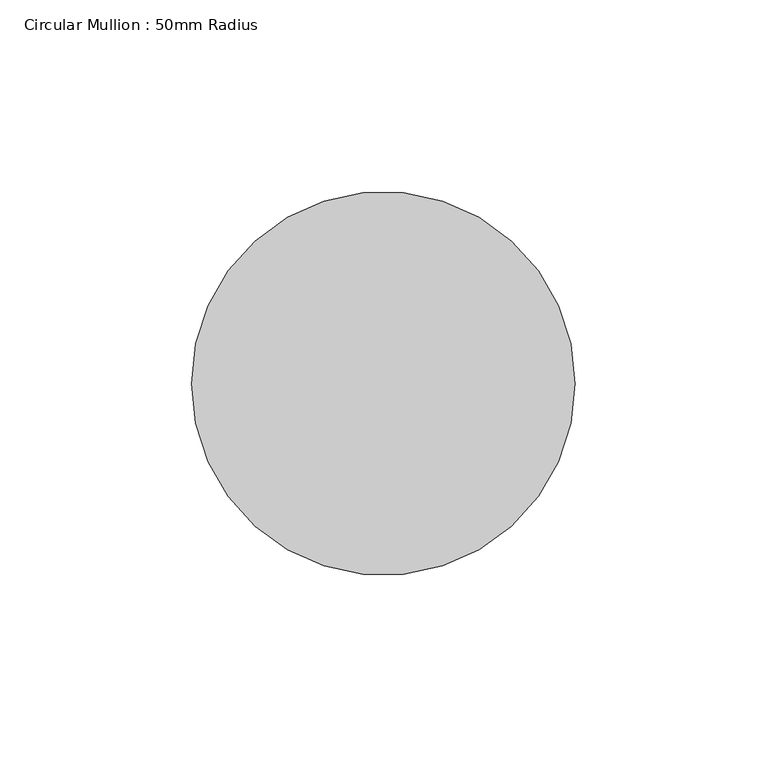
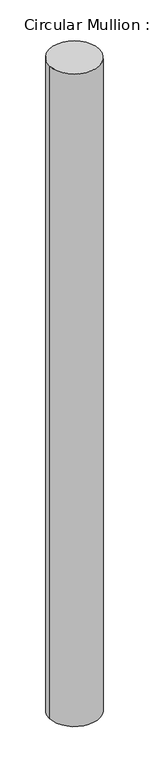
"""IFC4 building model written with IfcOpenShell, lengths in millimetres: member geometry, Circular Mullion : 50mm Radius."""

import ifcopenshell
import ifcopenshell.guid

model = None  # the IFC model being written
_history = None  # IfcOwnerHistory: only IFC2X3 demands one
_inside = {}  # id of a spatial element -> (the spatial element, [elements in it])
_under = {}  # id of a project, library or spatial element -> (it, [spatial elements below it])
_declared = {}  # id of a project -> (the project, [libraries it declares])
_typed = {}  # id of a type object -> (the type object, [elements of that type])
_made_of = {}  # id of a material, layer set ... -> (it, [elements and type objects made of it])


def new_model(schema):
    """Start an empty IFC model of exactly this schema.

    Asked for "IFC4X3", IfcOpenShell would pick the latest addendum, in which some entities
    have other attributes; the version numbers below select the first issue.
    IFC2X3 requires an IfcOwnerHistory on every rooted entity: one is made here for all.
    """
    global model, _history
    if schema == "IFC4X3":
        model = ifcopenshell.file(schema_version=(4, 3, 0, 0))
    else:
        model = ifcopenshell.file(schema=schema)
    _inside.clear()
    _under.clear()
    _declared.clear()
    _typed.clear()
    _made_of.clear()
    _history = None
    if model.schema == "IFC2X3":
        org = make("IfcOrganization", Name="unknown")
        user = make(
            "IfcPersonAndOrganization",
            ThePerson=make("IfcPerson", FamilyName="unknown"),
            TheOrganization=org,
        )
        app = make(
            "IfcApplication",
            ApplicationDeveloper=org,
            Version="unknown",
            ApplicationFullName="unknown",
            ApplicationIdentifier="unknown",
        )
        _history = make(
            "IfcOwnerHistory",
            OwningUser=user,
            OwningApplication=app,
            ChangeAction="ADDED",
            CreationDate=0,
        )
    return model


def make(cls, **values):
    """One entity of the class cls with the attributes given. An attribute that is None is left unset."""
    return model.create_entity(
        cls, **{name: value for name, value in values.items() if value is not None}
    )


def rooted(cls, **values):
    """An entity with a GlobalId (a new one), such as an element, a storey or a relation."""
    return make(cls, GlobalId=ifcopenshell.guid.new(), OwnerHistory=_history, **values)


def si_unit(unit_type, name, prefix=None):
    """IfcSIUnit, for example si_unit("LENGTHUNIT", "METRE", prefix="MILLI")."""
    return make("IfcSIUnit", UnitType=unit_type, Prefix=prefix, Name=name)


def assignment(units):
    """IfcUnitAssignment: the units of a project."""
    return None if units is None else make("IfcUnitAssignment", Units=units)


def point(xyz):
    """IfcCartesianPoint."""
    return None if xyz is None else make("IfcCartesianPoint", Coordinates=xyz)


def direction(xyz):
    """IfcDirection."""
    return None if xyz is None else make("IfcDirection", DirectionRatios=xyz)


def frame(location, z_axis=None, x_axis=None):
    """IfcAxis2Placement3D, a coordinate frame: its origin and axes. An axis left out is left unset."""
    return make(
        "IfcAxis2Placement3D",
        Location=point(location),
        Axis=direction(z_axis),
        RefDirection=direction(x_axis),
    )


def frame_2d(location, x_axis=None):
    """IfcAxis2Placement2D, a coordinate frame in the plane: its origin and x axis."""
    return make(
        "IfcAxis2Placement2D", Location=point(location), RefDirection=direction(x_axis)
    )


def origin():
    """The frame at (0, 0, 0) with its axes left unset."""
    return frame((0.0, 0.0, 0.0))


def origin_2d():
    """The frame at (0, 0) in the plane with its x axis left unset."""
    return frame_2d((0.0, 0.0))


def place(relative_to, where):
    """IfcLocalPlacement: puts the frame where relative to a parent placement (None: the world)."""
    return make(
        "IfcLocalPlacement", PlacementRelTo=relative_to, RelativePlacement=where
    )


def context(
    kind, dimensions, precision=None, world=None, true_north=None, identifier=None
):
    """IfcGeometricRepresentationContext, for example the 3D "Model" context."""
    return make(
        "IfcGeometricRepresentationContext",
        ContextIdentifier=identifier,
        ContextType=kind,
        CoordinateSpaceDimension=dimensions,
        Precision=precision,
        WorldCoordinateSystem=world,
        TrueNorth=true_north,
    )


def project(units=None, contexts=None):
    """IfcProject with its units and contexts."""
    return rooted(
        "IfcProject",
        Name="project",
        RepresentationContexts=contexts,
        UnitsInContext=assignment(units),
    )


def spatial(cls, under=None, at=None, **own):
    """A site, building, storey or space (cls), placed at a placement, below another one or the project."""
    s = rooted(cls, ObjectPlacement=at, **own)
    if under is not None:
        _under.setdefault(under.id(), (under, []))[1].append(s)
    return s


def circle_curve(where, radius):
    """IfcCircle in the frame where."""
    return make("IfcCircle", Position=where, Radius=radius)


def trimmed(basis, trim1, trim2, sense, master):
    """IfcTrimmedCurve: the piece of a basis curve between two trims."""
    return make(
        "IfcTrimmedCurve",
        BasisCurve=basis,
        Trim1=trim1,
        Trim2=trim2,
        SenseAgreement=sense,
        MasterRepresentation=master,
    )


def segment(curve, same_sense, transition):
    """IfcCompositeCurveSegment."""
    return make(
        "IfcCompositeCurveSegment",
        Transition=transition,
        SameSense=same_sense,
        ParentCurve=curve,
    )


def composite_curve(segments, self_intersect=None):
    """IfcCompositeCurve: segments joined end to end."""
    return make("IfcCompositeCurve", Segments=segments, SelfIntersect=self_intersect)


def outline(outer, holes=None, kind="AREA"):
    """IfcArbitraryClosedProfileDef: a profile drawn as a closed curve; with holes, ...WithVoids."""
    if holes is None:
        return make("IfcArbitraryClosedProfileDef", ProfileType=kind, OuterCurve=outer)
    return make(
        "IfcArbitraryProfileDefWithVoids",
        ProfileType=kind,
        OuterCurve=outer,
        InnerCurves=holes,
    )


def extrude(swept, where, along, depth):
    """IfcExtrudedAreaSolid: the profile swept, set in the frame where, extruded along a direction by depth."""
    return make(
        "IfcExtrudedAreaSolid",
        SweptArea=swept,
        Position=where,
        ExtrudedDirection=direction(along),
        Depth=depth,
    )


def shape(context_of_items, identifier, shape_type, items):
    """IfcShapeRepresentation: the items that make up one representation, for example the "Body"."""
    return make(
        "IfcShapeRepresentation",
        ContextOfItems=context_of_items,
        RepresentationIdentifier=identifier,
        RepresentationType=shape_type,
        Items=items,
    )


def source(mapping_origin, context_of_items, identifier, shape_type, items):
    """IfcRepresentationMap: a shape defined once, which mapped items show again and again."""
    return make(
        "IfcRepresentationMap",
        MappingOrigin=mapping_origin,
        MappedRepresentation=shape(context_of_items, identifier, shape_type, items),
    )


def transform(
    local_origin,
    x_axis=None,
    y_axis=None,
    z_axis=None,
    scale=None,
    scale2=None,
    scale3=None,
    uniform=True,
):
    """IfcCartesianTransformationOperator3D, or its non-uniform kind. x_axis, y_axis, z_axis: its Axis1, 2, 3."""
    if uniform:
        return make(
            "IfcCartesianTransformationOperator3D",
            Axis1=direction(x_axis),
            Axis2=direction(y_axis),
            LocalOrigin=point(local_origin),
            Scale=scale,
            Axis3=direction(z_axis),
        )
    return make(
        "IfcCartesianTransformationOperator3DnonUniform",
        Axis1=direction(x_axis),
        Axis2=direction(y_axis),
        LocalOrigin=point(local_origin),
        Scale=scale,
        Axis3=direction(z_axis),
        Scale2=scale2,
        Scale3=scale3,
    )


def mapped(mapping_source, mapping_target):
    """IfcMappedItem: shows the shape of a source again, moved by a transform."""
    return make(
        "IfcMappedItem", MappingSource=mapping_source, MappingTarget=mapping_target
    )


def made_of(thing, what):
    """Note that an element or type object is made of a material, layer set ...; save() writes the relation."""
    if what is not None:
        _made_of.setdefault(what.id(), (what, []))[1].append(thing)
    return thing


def element(
    cls,
    number,
    at=None,
    inside=None,
    cuts=None,
    type_object=None,
    material=None,
    context=None,
    identifier="Body",
    shape_type=None,
    held_by="IfcProductDefinitionShape",
    body=None,
    shapes=None,
    **own,
):
    """One element of the class cls, such as IfcWall. Its Tag is "e" and its number.

    at: its placement. inside: the storey or other place that contains it. cuts: it is an
    opening in that element (IfcRelVoidsElement). A single representation is given by context,
    identifier, shape_type and body (its items); several are given by shapes. held_by: the class
    of the entity that holds the representations. save() writes the other relations.
    """
    e = rooted(cls, Tag="e%d" % number, ObjectPlacement=at, **own)
    if body is not None:
        shapes = [shape(context, identifier, shape_type, body)]
    if shapes is not None:
        e.Representation = make(held_by, Representations=shapes)
    if inside is not None:
        _inside.setdefault(inside.id(), (inside, []))[1].append(e)
    if cuts is not None:
        rooted(
            "IfcRelVoidsElement", RelatingBuildingElement=cuts, RelatedOpeningElement=e
        )
    if type_object is not None:
        _typed.setdefault(type_object.id(), (type_object, []))[1].append(e)
    return made_of(e, material)


def aggregate(whole, parts):
    """IfcRelAggregates: a whole, such as a stair, and the parts it consists of."""
    return rooted("IfcRelAggregates", RelatingObject=whole, RelatedObjects=parts)


def save(model, path):
    """Write the relations noted so far, then the file.

    IfcRelAggregates (storeys below a building ...), IfcRelContainedInSpatialStructure (elements
    in a storey), IfcRelDefinesByType, IfcRelAssociatesMaterial and IfcRelDeclares: one each for
    every whole, place, type object, material and project.
    """
    for whole, parts in _under.values():
        aggregate(whole, parts)
    for where, things in _inside.values():
        rooted(
            "IfcRelContainedInSpatialStructure",
            RelatedElements=things,
            RelatingStructure=where,
        )
    for kind, things in _typed.values():
        rooted("IfcRelDefinesByType", RelatedObjects=things, RelatingType=kind)
    for what, things in _made_of.values():
        rooted("IfcRelAssociatesMaterial", RelatedObjects=things, RelatingMaterial=what)
    for by, libraries in _declared.values():
        rooted("IfcRelDeclares", RelatingContext=by, RelatedDefinitions=libraries)
    model.write(path)


def circular_mullion_50mm_radius_c1c88358(model_context):
    return source(origin(), model_context, "Body", "SweptSolid", [
        extrude(outline(composite_curve([segment(trimmed(circle_curve(origin_2d(), 50.0), [point((50.0, 0.0))], [point((-50.0, 0.0))], False, "CARTESIAN"), True, "CONTINUOUS"), segment(trimmed(circle_curve(origin_2d(), 50.0), [point((-50.0, 0.0))], [point((50.0, 0.0))], False, "CARTESIAN"), True, "CONTINUOUS")], self_intersect=False)), frame((0.0, 0.0, -1382.3476871), z_axis=(0.0, 0.0, 1.0), x_axis=(1.0, 0.0, 0.0)), (0.0, 0.0, 1.0), 1382.3476871),
    ])


if __name__ == "__main__":
    model = new_model("IFC4")
    model_context = context("Model", 3, world=origin())
    ifc_project = project(units=[si_unit("LENGTHUNIT", "METRE", prefix="MILLI")], contexts=[model_context])
    site = spatial("IfcSite", under=ifc_project)
    building = spatial("IfcBuilding", under=site)
    placement = place(None, origin())
    circular_mullion_50mm_radius_shape = circular_mullion_50mm_radius_c1c88358(model_context)
    element("IfcMember", 1, ObjectType="Circular Mullion : 50mm Radius", at=placement, inside=building, context=model_context, shape_type="MappedRepresentation", body=[
        mapped(circular_mullion_50mm_radius_shape, transform((0.0, 0.0, 0.0), x_axis=(1.0, 0.0, 0.0), y_axis=(0.0, 1.0, 0.0), z_axis=(0.0, 0.0, 1.0))),
    ])
    save(model, "model.ifc")

# Revit data of these elements
# Type "Circular Mullion : 50mm Radius"
#   built-in parameter 1007350 = 0.164042 (stored number, unit not read)
# Element 1 (IfcMember, "Circular Mullion : 50mm Radius")
#   Materials on its faces: "Aluminium"
# Materials
#   "Aluminium": class "Metal", colour RGB 247 247 247, transparency 0, Description = "Aluminium 6061", Cost = 0
